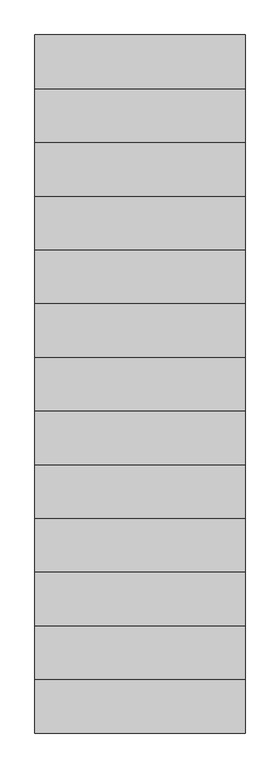
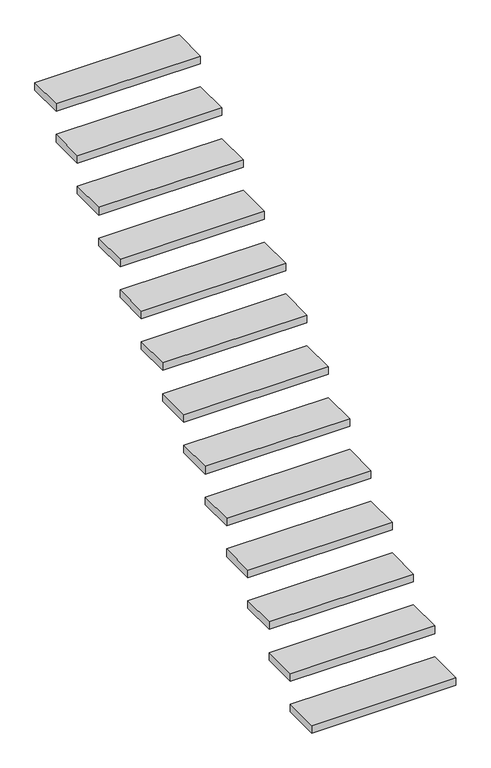
"""IFC4 building model written with IfcOpenShell, lengths in millimetres: stair geometry,   150414 :   150414."""

from ifc_helpers import new_model, si_unit, frame, origin, place, context, project, spatial, polyline, outline, extrude, source, transform, mapped, element, save


def stair_5d17669e(model_context):
    return source(origin(), model_context, "Body", "SweptSolid", [
        extrude(outline(polyline([(166797.7593015, 42144.7962965), (166797.7593015, 41914.7962965), (165897.7593015, 41914.7962965), (165897.7593015, 42144.7962965), (166797.7593015, 42144.7962965)])), frame((0.0, 0.0, 3482.1428571), z_axis=(0.0, 0.0, 1.0), x_axis=(1.0, 0.0, 0.0)), (0.0, 0.0, 1.0), 50.0),
        extrude(outline(polyline([(166797.7593015, 42374.7962965), (166797.7593015, 42144.7962965), (165897.7593015, 42144.7962965), (165897.7593015, 42374.7962965), (166797.7593015, 42374.7962965)])), frame((0.0, 0.0, 3684.2857143), z_axis=(0.0, 0.0, 1.0), x_axis=(1.0, 0.0, 0.0)), (0.0, 0.0, 1.0), 50.0),
        extrude(outline(polyline([(166797.7593015, 42604.7962965), (166797.7593015, 42374.7962965), (165897.7593015, 42374.7962965), (165897.7593015, 42604.7962965), (166797.7593015, 42604.7962965)])), frame((0.0, 0.0, 3886.4285714), z_axis=(0.0, 0.0, 1.0), x_axis=(1.0, 0.0, 0.0)), (0.0, 0.0, 1.0), 50.0),
        extrude(outline(polyline([(166797.7593015, 42834.7962965), (166797.7593015, 42604.7962965), (165897.7593015, 42604.7962965), (165897.7593015, 42834.7962965), (166797.7593015, 42834.7962965)])), frame((0.0, 0.0, 4088.5714286), z_axis=(0.0, 0.0, 1.0), x_axis=(1.0, 0.0, 0.0)), (0.0, 0.0, 1.0), 50.0),
        extrude(outline(polyline([(166797.7593015, 43064.7962965), (166797.7593015, 42834.7962965), (165897.7593015, 42834.7962965), (165897.7593015, 43064.7962965), (166797.7593015, 43064.7962965)])), frame((0.0, 0.0, 4290.7142857), z_axis=(0.0, 0.0, 1.0), x_axis=(1.0, 0.0, 0.0)), (0.0, 0.0, 1.0), 50.0),
        extrude(outline(polyline([(166797.7593015, 43294.7962965), (166797.7593015, 43064.7962965), (165897.7593015, 43064.7962965), (165897.7593015, 43294.7962965), (166797.7593015, 43294.7962965)])), frame((0.0, 0.0, 4492.8571429), z_axis=(0.0, 0.0, 1.0), x_axis=(1.0, 0.0, 0.0)), (0.0, 0.0, 1.0), 50.0),
        extrude(outline(polyline([(166797.7593015, 43524.7962965), (166797.7593015, 43294.7962965), (165897.7593015, 43294.7962965), (165897.7593015, 43524.7962965), (166797.7593015, 43524.7962965)])), frame((0.0, 0.0, 4695.0), z_axis=(0.0, 0.0, 1.0), x_axis=(1.0, 0.0, 0.0)), (0.0, 0.0, 1.0), 50.0),
        extrude(outline(polyline([(166797.7593015, 43754.7962965), (166797.7593015, 43524.7962965), (165897.7593015, 43524.7962965), (165897.7593015, 43754.7962965), (166797.7593015, 43754.7962965)])), frame((0.0, 0.0, 4897.1428571), z_axis=(0.0, 0.0, 1.0), x_axis=(1.0, 0.0, 0.0)), (0.0, 0.0, 1.0), 50.0),
        extrude(outline(polyline([(166797.7593015, 43984.7962965), (166797.7593015, 43754.7962965), (165897.7593015, 43754.7962965), (165897.7593015, 43984.7962965), (166797.7593015, 43984.7962965)])), frame((0.0, 0.0, 5099.2857143), z_axis=(0.0, 0.0, 1.0), x_axis=(1.0, 0.0, 0.0)), (0.0, 0.0, 1.0), 50.0),
        extrude(outline(polyline([(166797.7593015, 44214.7962965), (166797.7593015, 43984.7962965), (165897.7593015, 43984.7962965), (165897.7593015, 44214.7962965), (166797.7593015, 44214.7962965)])), frame((0.0, 0.0, 5301.4285714), z_axis=(0.0, 0.0, 1.0), x_axis=(1.0, 0.0, 0.0)), (0.0, 0.0, 1.0), 50.0),
        extrude(outline(polyline([(166797.7593015, 44444.7962965), (166797.7593015, 44214.7962965), (165897.7593015, 44214.7962965), (165897.7593015, 44444.7962965), (166797.7593015, 44444.7962965)])), frame((0.0, 0.0, 5503.5714286), z_axis=(0.0, 0.0, 1.0), x_axis=(1.0, 0.0, 0.0)), (0.0, 0.0, 1.0), 50.0),
        extrude(outline(polyline([(166797.7593015, 44674.7962965), (166797.7593015, 44444.7962965), (165897.7593015, 44444.7962965), (165897.7593015, 44674.7962965), (166797.7593015, 44674.7962965)])), frame((0.0, 0.0, 5705.7142857), z_axis=(0.0, 0.0, 1.0), x_axis=(1.0, 0.0, 0.0)), (0.0, 0.0, 1.0), 50.0),
        extrude(outline(polyline([(166797.7593015, 44904.7962965), (166797.7593015, 44674.7962965), (165897.7593015, 44674.7962965), (165897.7593015, 44904.7962965), (166797.7593015, 44904.7962965)])), frame((0.0, 0.0, 5907.8571429), z_axis=(0.0, 0.0, 1.0), x_axis=(1.0, 0.0, 0.0)), (0.0, 0.0, 1.0), 50.0),
    ])


if __name__ == "__main__":
    model = new_model("IFC4")
    model_context = context("Model", 3, world=origin())
    ifc_project = project(units=[si_unit("LENGTHUNIT", "METRE", prefix="MILLI")], contexts=[model_context])
    site = spatial("IfcSite", under=ifc_project)
    building = spatial("IfcBuilding", under=site)
    placement = place(None, origin())
    stair_shape = stair_5d17669e(model_context)
    element("IfcStair", 1, ObjectType="  150414 :   150414", at=placement, inside=building, context=model_context, shape_type="MappedRepresentation", body=[
        mapped(stair_shape, transform((0.0, 0.0, 0.0), x_axis=(1.0, 0.0, 0.0), y_axis=(0.0, 1.0, 0.0), z_axis=(0.0, 0.0, 1.0))),
    ])
    save(model, "model.ifc")

# Revit data of these elements
# Type "  150414 :   150414"
#   Abrechnungsart = "St"
#   Allright_Bauteil_ID = "0131Tre0659044575"
#   Codetext = "TR-MASSIV-GER\\"
#   Material = "Stahlbeton"
#   Objektname = "Treppe"
#   NameOverride = " "
#   Reference = "STB-Treppe"
#   ThermalTransmittance = 0.0000 BTU/(h·ft²·°F)
#   NosingLength = 0.000 m
#   NumberOfRiser = 14
#   NumberOfTreads = 13
#   RiserHeight = 2.021 m
#   TreadLength = 2.300 m
#   IsExternal = no
#   FireExit = no
#   HandicapAccessible = no
#   HasNonSkidSurface = no
# Element 1 (IfcStair, "  150414 :   150414")
#   Materials on its faces: "weiss"
# Materials
#   "weiss": class "Unassigned", colour RGB 255 255 255, transparency 0
